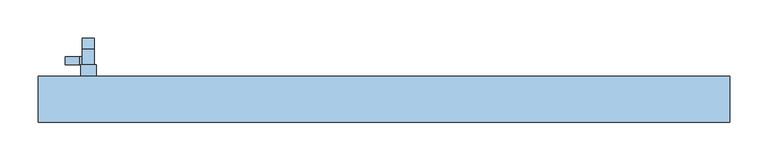
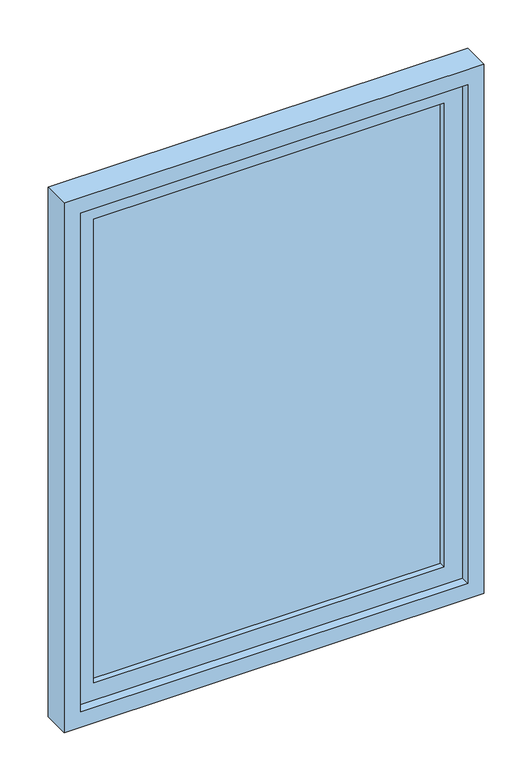
"""IFC4 building model written with IfcOpenShell, lengths in millimetres: window geometry, Inclinar e virar janela - 1 Painel : Inclinar e virar janela - 1 Painel."""

from ifc_helpers import new_model, si_unit, point, frame, frame_2d, origin, place, context, project, spatial, polyline, circle_curve, trimmed, segment, composite_curve, outline, extrude, source, transform, mapped, element, save


def window_cb8df3df(model_context):
    return source(origin(), model_context, "Body", "SweptSolid", [
        extrude(outline(composite_curve([segment(polyline([(95.0, 1259.0), (85.0, 1259.0), (85.0, 1277.0), (105.0, 1277.0)]), True, "CONTINUOUS"), segment(trimmed(circle_curve(frame_2d((105.0, 1263.0)), 14.0), [point((105.0, 1277.0))], [point((119.0, 1263.0))], False, "CARTESIAN"), True, "CONTINUOUS"), segment(polyline([(119.0, 1263.0), (119.0, 1120.0), (114.0, 1120.0), (106.9888756, 1235.3294081)]), True, "CONTINUOUS"), segment(trimmed(circle_curve(frame_2d((100.9630874, 1234.9630874)), 6.0369126), [point((106.9888756, 1235.3294081))], [point((100.9630874, 1241.0))], True, "CARTESIAN"), True, "CONTINUOUS"), segment(polyline([(100.9630874, 1241.0), (95.0, 1241.0), (95.0, 1259.0)]), True, "CONTINUOUS")], self_intersect=False)), frame((-393.0, 0.0, 0.0), z_axis=(1.0, 0.0, 0.0), x_axis=(0.0, 1.0, 0.0)), (0.0, 0.0, 1.0), 16.0),
        extrude(outline(polyline([(1259.0, -377.0), (1259.0, -396.9864015), (1257.0348924, -415.0), (1243.0157191, -415.0), (1241.0, -396.9864015), (1241.0, -377.0), (1259.0, -377.0)])), frame((0.0, 85.0, 0.0), z_axis=(0.0, 1.0, 0.0), x_axis=(0.0, 0.0, 1.0)), (0.0, 0.0, 1.0), 10.0),
        extrude(outline(polyline([(-395.0, 85.0), (-375.0, 85.0), (-375.0, 70.0), (-395.0, 70.0), (-395.0, 85.0)])), frame((0.0, 0.0, 1218.0), z_axis=(0.0, 0.0, 1.0), x_axis=(1.0, 0.0, 0.0)), (0.0, 0.0, 1.0), 64.0),
        extrude(outline(polyline([(375.0, 43.0), (-375.0, 43.0), (-375.0, 57.0), (375.0, 57.0), (375.0, 43.0)])), frame((0.0, 0.0, 725.0), z_axis=(0.0, 0.0, 1.0), x_axis=(1.0, 0.0, 0.0)), (0.0, 0.0, 1.0), 1050.0),
        extrude(outline(polyline([(1815.0, -415.0), (685.0, -415.0), (685.0, 415.0), (1815.0, 415.0), (1815.0, -415.0)]), holes=[polyline([(725.0, -375.0), (1775.0, -375.0), (1775.0, 375.0), (725.0, 375.0), (725.0, -375.0)])]), frame((0.0, 30.0, 0.0), z_axis=(0.0, 1.0, 0.0), x_axis=(0.0, 0.0, 1.0)), (0.0, 0.0, 1.0), 40.0),
        extrude(outline(polyline([(1850.0, -450.0), (650.0, -450.0), (650.0, 450.0), (1850.0, 450.0), (1850.0, -450.0)]), holes=[polyline([(685.0, -415.0), (1815.0, -415.0), (1815.0, 415.0), (685.0, 415.0), (685.0, -415.0)])]), frame((0.0, 10.0, 0.0), z_axis=(0.0, 1.0, 0.0), x_axis=(0.0, 0.0, 1.0)), (0.0, 0.0, 1.0), 60.0),
    ])


if __name__ == "__main__":
    model = new_model("IFC4")
    model_context = context("Model", 3, world=origin())
    ifc_project = project(units=[si_unit("LENGTHUNIT", "METRE", prefix="MILLI")], contexts=[model_context])
    site = spatial("IfcSite", under=ifc_project)
    building = spatial("IfcBuilding", under=site)
    placement = place(None, origin())
    window_shape = window_cb8df3df(model_context)
    element("IfcWindow", 1, ObjectType="Inclinar e virar janela - 1 Painel : Inclinar e virar janela - 1 Painel", at=placement, inside=building, context=model_context, shape_type="MappedRepresentation", body=[
        mapped(window_shape, transform((0.0, 0.0, 0.0), x_axis=(1.0, 0.0, 0.0), y_axis=(0.0, 1.0, 0.0), z_axis=(0.0, 0.0, 1.0))),
    ])
    save(model, "model.ifc")

# Revit data of these elements
# Type "Inclinar e virar janela - 1 Painel : Inclinar e virar janela - 1 Painel"
#   Type Mark = "EF28"
#   Construction Type Id = "SGL"
#   Analytic Construction = "Janelas grandes envidraçadas únicas"
#   W1 = 0.830 m
#   Visual Light Transmittance = 0.9
#   Solar Heat Gain Coefficient = 0.86
#   Rough Width = 0.900 m
#   Rough Height = 1.200 m
#   Largura da moldura do painel = 0.040 m
#   Espessura da moldura do painel = 0.040 m
#   Height = 1.200 m
#   Heat Transfer Coefficient (U) = 5.5617 W/(m²·K)
#   H1 = 1.130 m
#   Largura da estrutura = 0.035 m
#   Espessura da moldura = 0.060 m
#   Altura-padrão do peitoril = 0.650 m
#   Width = 0.900 m
#   Define Thermal Properties by = 1
#   Material do puxador = none
#   Vidro = none
#   Material da moldura = none
#   Wall Closure = (empty or 0)
# Element 1 (IfcWindow, "Inclinar e virar janela - 1 Painel : Inclinar e virar janela - 1 Painel")
#   Materials on its faces: "Glass"
# Materials
#   "Glass": class "Glass", colour RGB 0 128 192, transparency 0.75, Description = "Soda Lime Glass", Cost = 0
